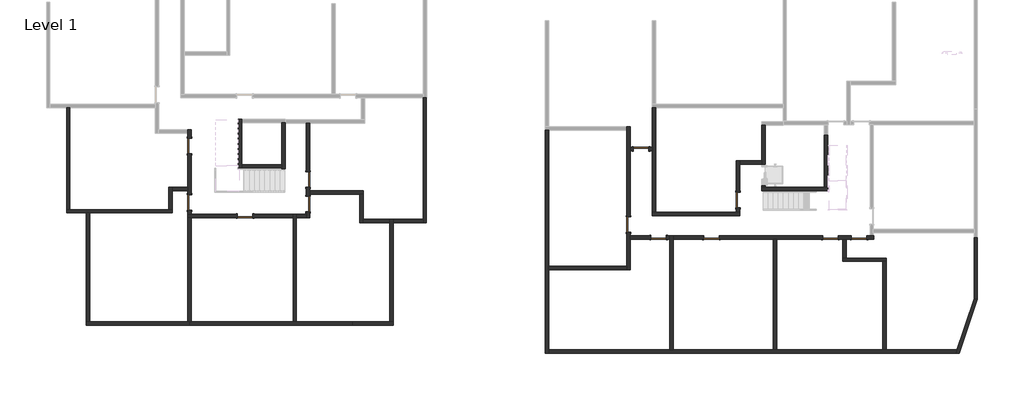
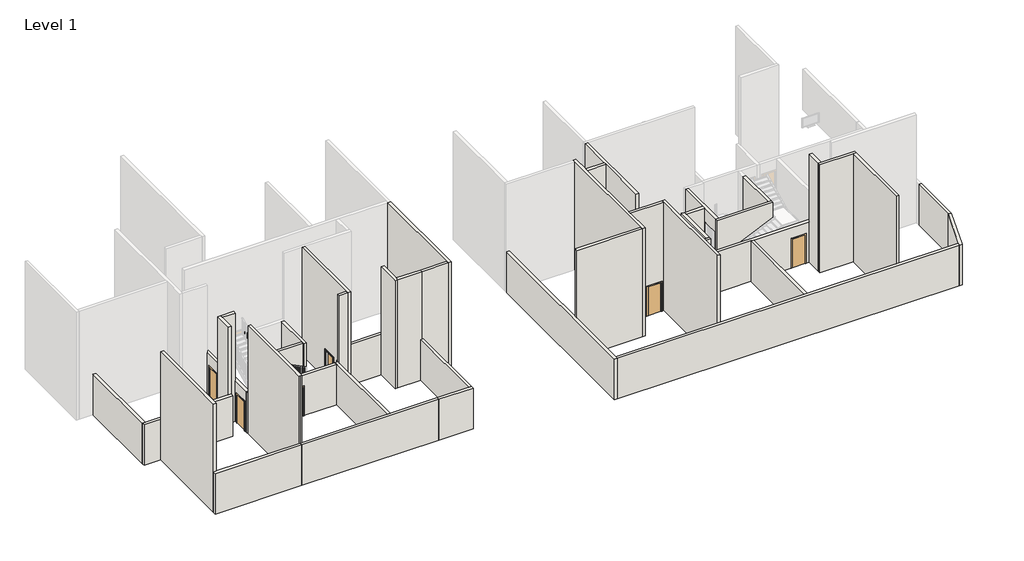
# One storey, part 1 of 3: 44 walls, 12 doors.
"""IFC4 building model written with IfcOpenShell, lengths in millimetres."""

import ifcopenshell
import ifcopenshell.guid

model = None  # the IFC model being written
_history = None  # IfcOwnerHistory: only IFC2X3 demands one
_inside = {}  # id of a spatial element -> (the spatial element, [elements in it])
_under = {}  # id of a project, library or spatial element -> (it, [spatial elements below it])
_declared = {}  # id of a project -> (the project, [libraries it declares])
_typed = {}  # id of a type object -> (the type object, [elements of that type])
_made_of = {}  # id of a material, layer set ... -> (it, [elements and type objects made of it])


def new_model(schema):
    """Start an empty IFC model of exactly this schema.

    Asked for "IFC4X3", IfcOpenShell would pick the latest addendum, in which some entities
    have other attributes; the version numbers below select the first issue.
    IFC2X3 requires an IfcOwnerHistory on every rooted entity: one is made here for all.
    """
    global model, _history
    if schema == "IFC4X3":
        model = ifcopenshell.file(schema_version=(4, 3, 0, 0))
    else:
        model = ifcopenshell.file(schema=schema)
    _inside.clear()
    _under.clear()
    _declared.clear()
    _typed.clear()
    _made_of.clear()
    _history = None
    if model.schema == "IFC2X3":
        org = make("IfcOrganization", Name="unknown")
        user = make(
            "IfcPersonAndOrganization",
            ThePerson=make("IfcPerson", FamilyName="unknown"),
            TheOrganization=org,
        )
        app = make(
            "IfcApplication",
            ApplicationDeveloper=org,
            Version="unknown",
            ApplicationFullName="unknown",
            ApplicationIdentifier="unknown",
        )
        _history = make(
            "IfcOwnerHistory",
            OwningUser=user,
            OwningApplication=app,
            ChangeAction="ADDED",
            CreationDate=0,
        )
    return model


def make(cls, **values):
    """One entity of the class cls with the attributes given. An attribute that is None is left unset."""
    return model.create_entity(
        cls, **{name: value for name, value in values.items() if value is not None}
    )


def rooted(cls, **values):
    """An entity with a GlobalId (a new one), such as an element, a storey or a relation."""
    return make(cls, GlobalId=ifcopenshell.guid.new(), OwnerHistory=_history, **values)


def si_unit(unit_type, name, prefix=None):
    """IfcSIUnit, for example si_unit("LENGTHUNIT", "METRE", prefix="MILLI")."""
    return make("IfcSIUnit", UnitType=unit_type, Prefix=prefix, Name=name)


def assignment(units):
    """IfcUnitAssignment: the units of a project."""
    return None if units is None else make("IfcUnitAssignment", Units=units)


def point(xyz):
    """IfcCartesianPoint."""
    return None if xyz is None else make("IfcCartesianPoint", Coordinates=xyz)


def direction(xyz):
    """IfcDirection."""
    return None if xyz is None else make("IfcDirection", DirectionRatios=xyz)


def frame(location, z_axis=None, x_axis=None):
    """IfcAxis2Placement3D, a coordinate frame: its origin and axes. An axis left out is left unset."""
    return make(
        "IfcAxis2Placement3D",
        Location=point(location),
        Axis=direction(z_axis),
        RefDirection=direction(x_axis),
    )


def origin():
    """The frame at (0, 0, 0) with its axes left unset."""
    return frame((0.0, 0.0, 0.0))


def origin_with_axes():
    """The frame at (0, 0, 0) with the z axis (0, 0, 1) and the x axis (1, 0, 0) written out."""
    return frame((0.0, 0.0, 0.0), z_axis=(0.0, 0.0, 1.0), x_axis=(1.0, 0.0, 0.0))


def place(relative_to, where):
    """IfcLocalPlacement: puts the frame where relative to a parent placement (None: the world)."""
    return make(
        "IfcLocalPlacement", PlacementRelTo=relative_to, RelativePlacement=where
    )


def context(
    kind, dimensions, precision=None, world=None, true_north=None, identifier=None
):
    """IfcGeometricRepresentationContext, for example the 3D "Model" context."""
    return make(
        "IfcGeometricRepresentationContext",
        ContextIdentifier=identifier,
        ContextType=kind,
        CoordinateSpaceDimension=dimensions,
        Precision=precision,
        WorldCoordinateSystem=world,
        TrueNorth=true_north,
    )


def project(units=None, contexts=None):
    """IfcProject with its units and contexts."""
    return rooted(
        "IfcProject",
        Name="project",
        RepresentationContexts=contexts,
        UnitsInContext=assignment(units),
    )


def spatial(cls, under=None, at=None, **own):
    """A site, building, storey or space (cls), placed at a placement, below another one or the project."""
    s = rooted(cls, ObjectPlacement=at, **own)
    if under is not None:
        _under.setdefault(under.id(), (under, []))[1].append(s)
    return s


def polyline(points):
    """IfcPolyline through the points."""
    return make("IfcPolyline", Points=[point(p) for p in points])


def outline(outer, holes=None, kind="AREA"):
    """IfcArbitraryClosedProfileDef: a profile drawn as a closed curve; with holes, ...WithVoids."""
    if holes is None:
        return make("IfcArbitraryClosedProfileDef", ProfileType=kind, OuterCurve=outer)
    return make(
        "IfcArbitraryProfileDefWithVoids",
        ProfileType=kind,
        OuterCurve=outer,
        InnerCurves=holes,
    )


def extrude(swept, where, along, depth):
    """IfcExtrudedAreaSolid: the profile swept, set in the frame where, extruded along a direction by depth."""
    return make(
        "IfcExtrudedAreaSolid",
        SweptArea=swept,
        Position=where,
        ExtrudedDirection=direction(along),
        Depth=depth,
    )


def faces_of(points, faces, orient=None, outer=None):
    """IfcFace entities. A face is a list of loops; a loop is a list of indices into points, from 0.

    orient and outer hold one flag for each loop. By default every Orientation is true, the
    first loop of a face is its IfcFaceOuterBound and the others are IfcFaceBound.
    """
    made = []
    for i, loops in enumerate(faces):
        bounds = []
        for j, loop in enumerate(loops):
            is_outer = j == 0 if outer is None else outer[i][j]
            bounds.append(
                make(
                    "IfcFaceOuterBound" if is_outer else "IfcFaceBound",
                    Bound=make("IfcPolyLoop", Polygon=[points[k] for k in loop]),
                    Orientation=True if orient is None else orient[i][j],
                )
            )
        made.append(make("IfcFace", Bounds=bounds))
    return made


def faceted_brep(points, faces, orient=None, outer=None, voids=None):
    """IfcFacetedBrep: a solid bounded by flat faces; with voids (closed shells), ...WithVoids."""
    shared = [point(p) for p in points]
    hull = make("IfcClosedShell", CfsFaces=faces_of(shared, faces, orient, outer))
    if voids is None:
        return make("IfcFacetedBrep", Outer=hull)
    return make(
        "IfcFacetedBrepWithVoids",
        Outer=hull,
        Voids=[
            make(cls, CfsFaces=faces_of(shared, fs, o, b)) for cls, fs, o, b in voids
        ],
    )


def shape(context_of_items, identifier, shape_type, items):
    """IfcShapeRepresentation: the items that make up one representation, for example the "Body"."""
    return make(
        "IfcShapeRepresentation",
        ContextOfItems=context_of_items,
        RepresentationIdentifier=identifier,
        RepresentationType=shape_type,
        Items=items,
    )


def source(mapping_origin, context_of_items, identifier, shape_type, items):
    """IfcRepresentationMap: a shape defined once, which mapped items show again and again."""
    return make(
        "IfcRepresentationMap",
        MappingOrigin=mapping_origin,
        MappedRepresentation=shape(context_of_items, identifier, shape_type, items),
    )


def transform(
    local_origin,
    x_axis=None,
    y_axis=None,
    z_axis=None,
    scale=None,
    scale2=None,
    scale3=None,
    uniform=True,
):
    """IfcCartesianTransformationOperator3D, or its non-uniform kind. x_axis, y_axis, z_axis: its Axis1, 2, 3."""
    if uniform:
        return make(
            "IfcCartesianTransformationOperator3D",
            Axis1=direction(x_axis),
            Axis2=direction(y_axis),
            LocalOrigin=point(local_origin),
            Scale=scale,
            Axis3=direction(z_axis),
        )
    return make(
        "IfcCartesianTransformationOperator3DnonUniform",
        Axis1=direction(x_axis),
        Axis2=direction(y_axis),
        LocalOrigin=point(local_origin),
        Scale=scale,
        Axis3=direction(z_axis),
        Scale2=scale2,
        Scale3=scale3,
    )


def mapped(mapping_source, mapping_target):
    """IfcMappedItem: shows the shape of a source again, moved by a transform."""
    return make(
        "IfcMappedItem", MappingSource=mapping_source, MappingTarget=mapping_target
    )


def made_of(thing, what):
    """Note that an element or type object is made of a material, layer set ...; save() writes the relation."""
    if what is not None:
        _made_of.setdefault(what.id(), (what, []))[1].append(thing)
    return thing


def element(
    cls,
    number,
    at=None,
    inside=None,
    cuts=None,
    type_object=None,
    material=None,
    context=None,
    identifier="Body",
    shape_type=None,
    held_by="IfcProductDefinitionShape",
    body=None,
    shapes=None,
    **own,
):
    """One element of the class cls, such as IfcWall. Its Tag is "e" and its number.

    at: its placement. inside: the storey or other place that contains it. cuts: it is an
    opening in that element (IfcRelVoidsElement). A single representation is given by context,
    identifier, shape_type and body (its items); several are given by shapes. held_by: the class
    of the entity that holds the representations. save() writes the other relations.
    """
    e = rooted(cls, Tag="e%d" % number, ObjectPlacement=at, **own)
    if body is not None:
        shapes = [shape(context, identifier, shape_type, body)]
    if shapes is not None:
        e.Representation = make(held_by, Representations=shapes)
    if inside is not None:
        _inside.setdefault(inside.id(), (inside, []))[1].append(e)
    if cuts is not None:
        rooted(
            "IfcRelVoidsElement", RelatingBuildingElement=cuts, RelatedOpeningElement=e
        )
    if type_object is not None:
        _typed.setdefault(type_object.id(), (type_object, []))[1].append(e)
    return made_of(e, material)


def aggregate(whole, parts):
    """IfcRelAggregates: a whole, such as a stair, and the parts it consists of."""
    return rooted("IfcRelAggregates", RelatingObject=whole, RelatedObjects=parts)


def save(model, path):
    """Write the relations noted so far, then the file.

    IfcRelAggregates (storeys below a building ...), IfcRelContainedInSpatialStructure (elements
    in a storey), IfcRelDefinesByType, IfcRelAssociatesMaterial and IfcRelDeclares: one each for
    every whole, place, type object, material and project.
    """
    for whole, parts in _under.values():
        aggregate(whole, parts)
    for where, things in _inside.values():
        rooted(
            "IfcRelContainedInSpatialStructure",
            RelatedElements=things,
            RelatingStructure=where,
        )
    for kind, things in _typed.values():
        rooted("IfcRelDefinesByType", RelatedObjects=things, RelatingType=kind)
    for what, things in _made_of.values():
        rooted("IfcRelAssociatesMaterial", RelatedObjects=things, RelatingMaterial=what)
    for by, libraries in _declared.values():
        rooted("IfcRelDeclares", RelatingContext=by, RelatedDefinitions=libraries)
    model.write(path)


def m_single_flush_0915_x_2134mm_727434cd(model_context):
    return source(origin(), model_context, "Body", "SweptSolid", [
        extrude(outline(polyline([(2210.0, -533.5), (0.0, -533.5), (0.0, -457.5), (2134.0, -457.5), (2134.0, 457.5), (0.0, 457.5), (0.0, 533.5), (2210.0, 533.5), (2210.0, -533.5)])), frame((0.0, -125.0, 0.0), z_axis=(0.0, 1.0, 0.0), x_axis=(0.0, 0.0, 1.0)), (0.0, 0.0, 1.0), 25.0),
        extrude(outline(polyline([(2210.0, 533.5), (2210.0, -533.5), (0.0, -533.5), (0.0, -457.5), (2134.0, -457.5), (2134.0, 457.5), (0.0, 457.5), (0.0, 533.5), (2210.0, 533.5)])), frame((0.0, 100.0, 0.0), z_axis=(0.0, 1.0, 0.0), x_axis=(0.0, 0.0, 1.0)), (0.0, 0.0, 1.0), 25.0),
        extrude(outline(polyline([(457.5, -49.0), (457.5, -100.0), (-457.5, -100.0), (-457.5, -49.0), (457.5, -49.0)])), origin_with_axes(), (0.0, 0.0, 1.0), 2134.0),
    ])


def m_single_flush_0915_x_2134mm_6a9e8738(model_context):
    return source(origin(), model_context, "Body", "SweptSolid", [
        extrude(outline(polyline([(2210.0, -533.5), (0.0, -533.5), (0.0, -457.5), (2134.0, -457.5), (2134.0, 457.5), (0.0, 457.5), (0.0, 533.5), (2210.0, 533.5), (2210.0, -533.5)])), frame((0.0, 100.0, 0.0), z_axis=(0.0, 1.0, 0.0), x_axis=(0.0, 0.0, 1.0)), (0.0, 0.0, 1.0), 25.0),
        extrude(outline(polyline([(2210.0, 533.5), (2210.0, -533.5), (0.0, -533.5), (0.0, -457.5), (2134.0, -457.5), (2134.0, 457.5), (0.0, 457.5), (0.0, 533.5), (2210.0, 533.5)])), frame((0.0, -125.0, 0.0), z_axis=(0.0, 1.0, 0.0), x_axis=(0.0, 0.0, 1.0)), (0.0, 0.0, 1.0), 25.0),
        extrude(outline(polyline([(457.5, 49.0), (-457.5, 49.0), (-457.5, 100.0), (457.5, 100.0), (457.5, 49.0)])), origin_with_axes(), (0.0, 0.0, 1.0), 2134.0),
    ])


model = new_model("IFC4")

# Units and contexts
model_context = context("Model", 3, world=origin())
ifc_project = project(units=[si_unit("LENGTHUNIT", "METRE", prefix="MILLI")], contexts=[model_context])

# Site, building, storey
site = spatial("IfcSite", under=ifc_project)
building = spatial("IfcBuilding", under=site)
storey = spatial("IfcBuildingStorey", under=building, Name="Level 1", Elevation=0.0)

# Doors
placement = place(None, origin())
m_single_flush_0915_x_2134mm_shape = m_single_flush_0915_x_2134mm_727434cd(model_context)
element("IfcDoor", 1, ObjectType="M_Single-Flush : 0915 x 2134mm", at=placement, inside=storey, context=model_context, shape_type="MappedRepresentation", body=[
    mapped(m_single_flush_0915_x_2134mm_shape, transform((16170.6041014, -4023.024372, 0.0), x_axis=(0.0, -1.0, 0.0), y_axis=(1.0, 0.0, 0.0), z_axis=(0.0, 0.0, 1.0))),
])
element("IfcDoor", 2, ObjectType="M_Single-Flush : 0915 x 2134mm", at=placement, inside=storey, context=model_context, shape_type="MappedRepresentation", body=[
    mapped(m_single_flush_0915_x_2134mm_shape, transform((-9130.3629108, -4269.650264, 0.0), x_axis=(0.0, 1.0, 0.0), y_axis=(-1.0, 0.0, 0.0), z_axis=(0.0, 0.0, 1.0))),
])
element("IfcDoor", 3, ObjectType="M_Single-Flush : 0915 x 2134mm", at=placement, inside=storey, context=model_context, shape_type="MappedRepresentation", body=[
    mapped(m_single_flush_0915_x_2134mm_shape, transform((9728.8612349, -5479.1907835, 0.0), x_axis=(0.0, -1.0, 0.0), y_axis=(1.0, 0.0, 0.0), z_axis=(0.0, 0.0, 1.0))),
])
element("IfcDoor", 4, ObjectType="M_Single-Flush : 0915 x 2134mm", at=placement, inside=storey, context=model_context, shape_type="MappedRepresentation", body=[
    mapped(m_single_flush_0915_x_2134mm_shape, transform((21611.3612349, -6240.0098119, 0.0), x_axis=(1.0, 0.0, 0.0), y_axis=(0.0, 1.0, 0.0), z_axis=(0.0, 0.0, 1.0))),
])
element("IfcDoor", 5, ObjectType="M_Single-Flush : 0915 x 2134mm", at=placement, inside=storey, context=model_context, shape_type="MappedRepresentation", body=[
    mapped(m_single_flush_0915_x_2134mm_shape, transform((11502.336337, -6236.6907835, 0.0), x_axis=(1.0, 0.0, 0.0), y_axis=(0.0, 1.0, 0.0), z_axis=(0.0, 0.0, 1.0))),
])
m_single_flush_0915_x_2134mm_2_shape = m_single_flush_0915_x_2134mm_6a9e8738(model_context)
element("IfcDoor", 6, ObjectType="M_Single-Flush : 0915 x 2134mm", at=placement, inside=storey, context=model_context, shape_type="MappedRepresentation", body=[
    mapped(m_single_flush_0915_x_2134mm_2_shape, transform((14602.336337, -6240.0098119, 0.0), x_axis=(-1.0, 0.0, 0.0), y_axis=(0.0, -1.0, 0.0), z_axis=(0.0, 0.0, 1.0))),
])
element("IfcDoor", 7, ObjectType="M_Single-Flush : 0915 x 2134mm", at=placement, inside=storey, context=model_context, shape_type="MappedRepresentation", body=[
    mapped(m_single_flush_0915_x_2134mm_2_shape, transform((23308.8612349, -6240.0098119, 0.0), x_axis=(-1.0, 0.0, 0.0), y_axis=(0.0, -1.0, 0.0), z_axis=(0.0, 0.0, 1.0))),
])
element("IfcDoor", 8, ObjectType="M_Single-Flush : 0915 x 2134mm", at=placement, inside=storey, context=model_context, shape_type="MappedRepresentation", body=[
    mapped(m_single_flush_0915_x_2134mm_2_shape, transform((-12832.3304233, -4959.1627129, 0.0), x_axis=(-1.0, 0.0, 0.0), y_axis=(0.0, -1.0, 0.0), z_axis=(0.0, 0.0, 1.0))),
])
element("IfcDoor", 9, ObjectType="M_Single-Flush : 0915 x 2134mm", at=placement, inside=storey, context=model_context, shape_type="MappedRepresentation", body=[
    mapped(m_single_flush_0915_x_2134mm_2_shape, transform((-16113.9741722, -844.6599715, 0.0), x_axis=(0.0, 1.0, 0.0), y_axis=(-1.0, 0.0, 0.0), z_axis=(0.0, 0.0, 1.0))),
])
element("IfcDoor", 10, ObjectType="M_Single-Flush : 0915 x 2134mm", at=placement, inside=storey, context=model_context, shape_type="MappedRepresentation", body=[
    mapped(m_single_flush_0915_x_2134mm_2_shape, transform((-16113.9741722, -4173.1613422, 0.0), x_axis=(0.0, 1.0, 0.0), y_axis=(-1.0, 0.0, 0.0), z_axis=(0.0, 0.0, 1.0))),
])
element("IfcDoor", 11, ObjectType="M_Single-Flush : 0915 x 2134mm", at=placement, inside=storey, context=model_context, shape_type="MappedRepresentation", body=[
    mapped(m_single_flush_0915_x_2134mm_2_shape, transform((-9130.3629108, -2822.6378151, 0.0), x_axis=(0.0, -1.0, 0.0), y_axis=(1.0, 0.0, 0.0), z_axis=(0.0, 0.0, 1.0))),
])
element("IfcDoor", 12, ObjectType="M_Single-Flush : 0915 x 2134mm", at=placement, inside=storey, context=model_context, shape_type="MappedRepresentation", body=[
    mapped(m_single_flush_0915_x_2134mm_2_shape, transform((10478.8612349, -1020.524372, 0.0), x_axis=(1.0, 0.0, 0.0), y_axis=(0.0, 1.0, 0.0), z_axis=(0.0, 0.0, 1.0))),
])

# Walls
element("IfcWall", 13, ObjectType="Generic - 200mm", at=placement, inside=storey, context=model_context, shape_type="Brep", body=[
    faceted_brep([(30069.3799498, -6240.0098119, 0.0), (30069.3799498, -9831.8731192, 0.0), (30069.3799498, -9831.8731192, 3000.0), (30069.3799498, -6240.0098119, 3000.0), (30269.3799498, -6240.0098119, 0.0), (30269.3799498, -6240.0098119, 3000.0), (30269.3799498, -9864.7113693, 3000.0), (30269.3799498, -9864.7113693, 0.0), (30268.8612349, -6240.0098119, 0.0), (30268.8612349, -6240.0098119, 3000.0)], [[[0, 1, 2, 3]], [[4, 5, 6, 7]], [[1, 0, 8, 4, 7]], [[3, 2, 6, 5, 9]], [[0, 3, 9, 5, 4, 8]], [[2, 1, 7, 6]]]),
])
element("IfcWall", 14, ObjectType="Generic - 200mm", at=placement, inside=storey, context=model_context, shape_type="Brep", body=[
    faceted_brep([(21449.836337, -3276.2808257, 0.0), (21249.836337, -3276.2808257, 0.0), (17770.6041014, -3276.2808257, 0.0), (17570.6041014, -3276.2808257, 0.0), (17570.6041014, -3276.2808257, 3000.0), (17770.6041014, -3276.2808257, 3000.0), (21249.836337, -3276.2808257, 3000.0), (21449.836337, -3276.2808257, 3000.0), (21449.836337, -3476.2808257, 0.0), (21449.836337, -3476.2808257, 3000.0), (17570.6041014, -3476.2808257, 3000.0), (17570.6041014, -3476.2808257, 0.0)], [[[0, 1, 2, 3, 4, 5, 6, 7]], [[8, 9, 10, 11]], [[3, 2, 1, 0, 8, 11]], [[7, 6, 5, 4, 10, 9]], [[0, 7, 9, 8]], [[4, 3, 11, 10]]]),
])
element("IfcWall", 15, ObjectType="Generic - 200mm", at=placement, inside=storey, context=model_context, shape_type="SweptSolid", body=[
    extrude(outline(polyline([(18459.836337, -6340.0098119), (18459.836337, -12836.6907835), (18259.836337, -12836.6907835), (18259.836337, -6340.0098119), (18459.836337, -6340.0098119)])), origin_with_axes(), (0.0, 0.0, 1.0), 3000.0),
])
element("IfcWall", 16, ObjectType="Generic - 200mm", at=placement, inside=storey, context=model_context, shape_type="Brep", body=[
    faceted_brep([(29055.3124022, -12836.6907835, 0.0), (24888.8612349, -12836.6907835, 0.0), (24688.8612349, -12836.6907835, 0.0), (18459.836337, -12836.6907835, 0.0), (18259.836337, -12836.6907835, 0.0), (12359.836337, -12836.6907835, 0.0), (12159.836337, -12836.6907835, 0.0), (5043.716007, -12836.6907835, 0.0), (5043.716007, -12836.6907835, 3000.0), (18259.836337, -12836.6907835, 3000.0), (18459.836337, -12836.6907835, 3000.0), (29055.3124022, -12836.6907835, 3000.0), (28987.8162902, -13036.6907835, 0.0), (28987.8162902, -13036.6907835, 3000.0), (5043.716007, -13036.6907835, 3000.0), (5043.716007, -13036.6907835, 0.0)], [[[0, 1, 2, 3, 4, 5, 6, 7, 8, 9, 10, 11]], [[12, 13, 14, 15]], [[7, 6, 5, 4, 3, 2, 1, 0, 12, 15]], [[11, 10, 9, 8, 14, 13]], [[0, 11, 13, 12]], [[8, 7, 15, 14]]]),
])
element("IfcWall", 17, ObjectType="Generic - 200mm", at=placement, inside=storey, context=model_context, shape_type="Brep", body=[
    faceted_brep([(30069.3799498, -9831.8731192, 0.0), (29055.3124022, -12836.6907835, 0.0), (28987.8162902, -13036.6907835, 0.0), (28987.8162902, -13036.6907835, 3000.0), (29055.3124022, -12836.6907835, 3000.0), (30069.3799498, -9831.8731192, 3000.0), (30269.3799498, -9864.7113693, 0.0), (30269.3799498, -9864.7113693, 3000.0), (29198.8985612, -13036.6907835, 3000.0), (29198.8985612, -13036.6907835, 0.0)], [[[0, 1, 2, 3, 4, 5]], [[6, 7, 8, 9]], [[2, 1, 0, 6, 9]], [[5, 4, 3, 8, 7]], [[0, 5, 7, 6]], [[3, 2, 9, 8]]]),
])
element("IfcWall", 18, ObjectType="Generic - 200mm", at=placement, inside=storey, context=model_context, shape_type="Brep", body=[
    faceted_brep([(22851.3612349, -6140.0098119, 0.0), (22068.8612349, -6140.0098119, 0.0), (22068.8612349, -6140.0098119, 2134.0), (21153.8612349, -6140.0098119, 2134.0), (21153.8612349, -6140.0098119, 0.0), (15059.836337, -6140.0098119, 0.0), (15059.836337, -6140.0098119, 2134.0), (14144.836337, -6140.0098119, 2134.0), (14144.836337, -6140.0098119, 0.0), (12359.836337, -6140.0098119, 0.0), (12359.836337, -6140.0098119, 3000.0), (23948.8612349, -6140.0098119, 3000.0), (24148.8612349, -6140.0098119, 3000.0), (24163.3998354, -6140.0098119, 3000.0), (24163.3998354, -6140.0098119, 0.0), (24148.8612349, -6140.0098119, 0.0), (23948.8612349, -6140.0098119, 0.0), (23766.3612349, -6140.0098119, 0.0), (23766.3612349, -6140.0098119, 2134.0), (22851.3612349, -6140.0098119, 2134.0), (22068.8612349, -6340.0098119, 2134.0), (22068.8612349, -6340.0098119, 0.0), (22348.8612349, -6340.0098119, 0.0), (22548.8612349, -6340.0098119, 0.0), (22851.3612349, -6340.0098119, 0.0), (22851.3612349, -6340.0098119, 2134.0), (23766.3612349, -6340.0098119, 2134.0), (23766.3612349, -6340.0098119, 0.0), (24163.3998354, -6340.0098119, 0.0), (24163.3998354, -6340.0098119, 3000.0), (18459.836337, -6340.0098119, 3000.0), (18259.836337, -6340.0098119, 3000.0), (12359.836337, -6340.0098119, 3000.0), (12359.836337, -6340.0098119, 0.0), (14144.836337, -6340.0098119, 0.0), (14144.836337, -6340.0098119, 2134.0), (15059.836337, -6340.0098119, 2134.0), (15059.836337, -6340.0098119, 0.0), (18259.836337, -6340.0098119, 0.0), (18459.836337, -6340.0098119, 0.0), (21153.8612349, -6340.0098119, 0.0), (21153.8612349, -6340.0098119, 2134.0)], [[[0, 1, 2, 3, 4, 5, 6, 7, 8, 9, 10, 11, 12, 13, 14, 15, 16, 17, 18, 19]], [[20, 21, 22, 23, 24, 25, 26, 27, 28, 29, 30, 31, 32, 33, 34, 35, 36, 37, 38, 39, 40, 41]], [[33, 9, 8, 34]], [[17, 16, 15, 14, 28, 27]], [[40, 39, 38, 37, 5, 4]], [[24, 23, 22, 21, 1, 0]], [[13, 12, 11, 10, 32, 31, 30, 29]], [[14, 13, 29, 28]], [[7, 35, 34, 8]], [[36, 6, 5, 37]], [[6, 36, 35, 7]], [[25, 24, 0, 19]], [[26, 25, 19, 18]], [[27, 26, 18, 17]], [[10, 9, 33, 32]], [[2, 1, 21, 20]], [[3, 2, 20, 41]], [[4, 3, 41, 40]]]),
])
element("IfcWall", 19, ObjectType="Generic - 200mm", at=placement, inside=storey, context=model_context, shape_type="Brep", body=[
    faceted_brep([(4843.716007, 79.9901881, 0.0), (4843.716007, -13036.6907835, 0.0), (4843.716007, -13036.6907835, 3000.0), (4843.716007, 79.9901881, 3000.0), (5043.716007, 79.9901881, 0.0), (5043.716007, 79.9901881, 3000.0), (5043.716007, -12836.6907835, 3000.0), (5043.716007, -13036.6907835, 3000.0), (5043.716007, -13036.6907835, 0.0), (5043.716007, -12836.6907835, 0.0), (5043.716007, -8120.0098119, 0.0), (5043.716007, -7920.0098119, 0.0)], [[[0, 1, 2, 3]], [[4, 5, 6, 7, 8, 9, 10, 11]], [[1, 0, 4, 11, 10, 9, 8]], [[3, 2, 7, 6, 5]], [[2, 1, 8, 7]], [[0, 3, 5, 4]]]),
])
element("IfcWall", 20, ObjectType="Generic - 200mm", at=placement, inside=storey, context=model_context, shape_type="SweptSolid", body=[
    extrude(outline(polyline([(21249.836337, -3276.2808257), (21249.836337, -200.524372), (21449.836337, -200.524372), (21449.836337, -3276.2808257), (21249.836337, -3276.2808257)])), origin_with_axes(), (0.0, 0.0, 1.0), 3000.0),
])
element("IfcWall", 21, ObjectType="Generic - 200mm", at=placement, inside=storey, context=model_context, shape_type="Brep", body=[
    faceted_brep([(17570.6041014, -3276.2808257, 3000.0), (17570.6041014, -1920.524372, 3000.0), (17570.6041014, -1720.524372, 3000.0), (17570.6041014, 379.475628, 3000.0), (17570.6041014, 379.475628, 0.0), (17570.6041014, -1720.524372, 0.0), (17570.6041014, -1920.524372, 0.0), (17570.6041014, -1926.2808257, 0.0), (17570.6041014, -1926.2808257, 2000.0), (17570.6041014, -3181.2876228, 2000.0), (17570.6041014, -3181.2876228, 0.0), (17570.6041014, -3276.2808257, 0.0), (17770.6041014, 379.475628, 3000.0), (17770.6041014, -3276.2808257, 3000.0), (17770.6041014, -3276.2808257, 0.0), (17770.6041014, -3181.2876228, 0.0), (17770.6041014, -3181.2876228, 2000.0), (17770.6041014, -1926.2808257, 2000.0), (17770.6041014, -1926.2808257, 0.0), (17770.6041014, 379.475628, 0.0)], [[[0, 1, 2, 3, 4, 5, 6, 7, 8, 9, 10, 11]], [[12, 13, 14, 15, 16, 17, 18, 19]], [[14, 11, 10, 15]], [[4, 19, 18, 7, 6, 5]], [[3, 2, 1, 0, 13, 12]], [[0, 11, 14, 13]], [[9, 16, 15, 10]], [[17, 8, 7, 18]], [[8, 17, 16, 9]], [[4, 3, 12, 19]]]),
])
element("IfcWall", 22, ObjectType="Generic - 200mm", at=placement, inside=storey, context=model_context, shape_type="Brep", body=[
    faceted_brep([(11128.8612349, -4940.0098119, 0.0), (16270.6041014, -4940.0098119, 0.0), (16270.6041014, -4940.0098119, 3000.0), (11128.8612349, -4940.0098119, 3000.0), (11128.8612349, -4740.0098119, 0.0), (11128.8612349, -4740.0098119, 3000.0), (16070.6041014, -4740.0098119, 3000.0), (16270.6041014, -4740.0098119, 3000.0), (16270.6041014, -4740.0098119, 0.0), (16070.6041014, -4740.0098119, 0.0), (11328.8612349, -4740.0098119, 0.0)], [[[0, 1, 2, 3]], [[4, 5, 6, 7, 8, 9, 10]], [[1, 0, 4, 10, 9, 8]], [[3, 2, 7, 6, 5]], [[2, 1, 8, 7]], [[0, 3, 5, 4]]]),
])
element("IfcWall", 23, ObjectType="Generic - 200mm", at=placement, inside=storey, context=model_context, shape_type="Brep", body=[
    faceted_brep([(16270.6041014, -1720.524372, 3000.0), (16270.6041014, -1920.524372, 3000.0), (16270.6041014, -4740.0098119, 3000.0), (16270.6041014, -4740.0098119, 0.0), (16270.6041014, -4480.524372, 0.0), (16270.6041014, -4480.524372, 2134.0), (16270.6041014, -3565.524372, 2134.0), (16270.6041014, -3565.524372, 0.0), (16270.6041014, -1920.524372, 0.0), (16270.6041014, -1720.524372, 0.0), (16070.6041014, -4740.0098119, 3000.0), (16070.6041014, -1720.524372, 3000.0), (16070.6041014, -1720.524372, 0.0), (16070.6041014, -3565.524372, 0.0), (16070.6041014, -3565.524372, 2134.0), (16070.6041014, -4480.524372, 2134.0), (16070.6041014, -4480.524372, 0.0), (16070.6041014, -4740.0098119, 0.0)], [[[0, 1, 2, 3, 4, 5, 6, 7, 8, 9]], [[10, 11, 12, 13, 14, 15, 16, 17]], [[3, 17, 16, 4]], [[12, 9, 8, 7, 13]], [[2, 1, 0, 11, 10]], [[3, 2, 10, 17]], [[0, 9, 12, 11]], [[15, 5, 4, 16]], [[6, 14, 13, 7]], [[14, 6, 5, 15]]]),
])
element("IfcWall", 24, ObjectType="Generic - 200mm", at=placement, inside=storey, context=model_context, shape_type="SweptSolid", body=[
    extrude(outline(polyline([(17570.6041014, -1920.524372), (16270.6041014, -1920.524372), (16270.6041014, -1720.524372), (17570.6041014, -1720.524372), (17570.6041014, -1920.524372)])), origin_with_axes(), (0.0, 0.0, 1.0), 3000.0),
])
element("IfcWall", 25, ObjectType="Generic - 200mm", at=placement, inside=storey, context=model_context, shape_type="Brep", body=[
    faceted_brep([(22348.8612349, -7641.2808257, 0.0), (24688.8612349, -7641.2808257, 0.0), (24888.8612349, -7641.2808257, 0.0), (24888.8612349, -7641.2808257, 8000.0), (24688.8612349, -7641.2808257, 8000.0), (22348.8612349, -7641.2808257, 8000.0), (22348.8612349, -7441.2808257, 0.0), (22348.8612349, -7441.2808257, 8000.0), (22548.8612349, -7441.2808257, 8000.0), (24888.8612349, -7441.2808257, 8000.0), (24888.8612349, -7441.2808257, 0.0), (22548.8612349, -7441.2808257, 0.0)], [[[0, 1, 2, 3, 4, 5]], [[6, 7, 8, 9, 10, 11]], [[2, 1, 0, 6, 11, 10]], [[5, 4, 3, 9, 8, 7]], [[3, 2, 10, 9]], [[0, 5, 7, 6]]]),
])
element("IfcWall", 26, ObjectType="Generic - 200mm", at=placement, inside=storey, context=model_context, shape_type="SweptSolid", body=[
    extrude(outline(polyline([(24688.8612349, -12836.6907835), (24688.8612349, -7641.2808257), (24888.8612349, -7641.2808257), (24888.8612349, -12836.6907835), (24688.8612349, -12836.6907835)])), origin_with_axes(), (0.0, 0.0, 1.0), 8000.0),
])
element("IfcWall", 27, ObjectType="Generic - 200mm", at=placement, inside=storey, context=model_context, shape_type="SweptSolid", body=[
    extrude(outline(polyline([(22548.8612349, -6340.0098119), (22548.8612349, -7441.2808257), (22348.8612349, -7441.2808257), (22348.8612349, -6340.0098119), (22548.8612349, -6340.0098119)])), origin_with_axes(), (0.0, 0.0, 1.0), 8000.0),
])
element("IfcWall", 28, ObjectType="Generic - 200mm", at=placement, inside=storey, context=model_context, shape_type="Brep", body=[
    faceted_brep([(9628.8612349, -5936.6907835, 2134.0), (9628.8612349, -5936.6907835, 0.0), (9628.8612349, -7920.0098119, 0.0), (9628.8612349, -8120.0098119, 0.0), (9628.8612349, -8120.0098119, 8000.0), (9628.8612349, -7920.0098119, 8000.0), (9628.8612349, 79.9901881, 8000.0), (9628.8612349, 279.9901881, 8000.0), (9628.8612349, 279.9901881, 0.0), (9628.8612349, 79.9901881, 0.0), (9628.8612349, -5021.6907835, 0.0), (9628.8612349, -5021.6907835, 2134.0), (9828.8612349, -8120.0098119, 0.0), (9828.8612349, -6336.6907835, 0.0), (9828.8612349, -6136.6907835, 0.0), (9828.8612349, -5936.6907835, 0.0), (9828.8612349, -5936.6907835, 2134.0), (9828.8612349, -5021.6907835, 2134.0), (9828.8612349, -5021.6907835, 0.0), (9828.8612349, -1120.524372, 0.0), (9828.8612349, -920.524372, 0.0), (9828.8612349, 279.9901881, 0.0), (9828.8612349, 279.9901881, 8000.0), (9828.8612349, -920.524372, 8000.0), (9828.8612349, -1120.524372, 8000.0), (9828.8612349, -6136.6907835, 8000.0), (9828.8612349, -6336.6907835, 8000.0), (9828.8612349, -8120.0098119, 8000.0)], [[[0, 1, 2, 3, 4, 5, 6, 7, 8, 9, 10, 11]], [[12, 13, 14, 15, 16, 17, 18, 19, 20, 21, 22, 23, 24, 25, 26, 27]], [[10, 9, 8, 21, 20, 19, 18]], [[3, 2, 1, 15, 14, 13, 12]], [[7, 6, 5, 4, 27, 26, 25, 24, 23, 22]], [[8, 7, 22, 21]], [[4, 3, 12, 27]], [[16, 15, 1, 0]], [[17, 16, 0, 11]], [[18, 17, 11, 10]]]),
])
element("IfcWall", 29, ObjectType="Generic - 200mm", at=placement, inside=storey, context=model_context, shape_type="SweptSolid", body=[
    extrude(outline(polyline([(5043.716007, -7920.0098119), (9628.8612349, -7920.0098119), (9628.8612349, -8120.0098119), (5043.716007, -8120.0098119), (5043.716007, -7920.0098119)])), origin_with_axes(), (0.0, 0.0, 1.0), 8000.0),
])
element("IfcWall", 30, ObjectType="Generic - 200mm", at=placement, inside=storey, context=model_context, shape_type="Brep", body=[
    faceted_brep([(-4309.8304233, -5158.643998, 0.0), (-4309.8304233, -5358.643998, 0.0), (-4309.8304233, -11188.643998, 0.0), (-4309.8304233, -11188.643998, 3000.0), (-4309.8304233, -5358.643998, 3000.0), (-4309.8304233, -5158.643998, 3000.0), (-4109.8304233, -5158.643998, 0.0), (-4109.8304233, -5158.643998, 3000.0), (-4109.8304233, -5358.643998, 3000.0), (-4109.8304233, -11188.643998, 3000.0), (-4109.8304233, -11188.643998, 0.0), (-4109.8304233, -5358.643998, 0.0), (-4209.8304233, -5158.643998, 3000.0)], [[[0, 1, 2, 3, 4, 5]], [[6, 7, 8, 9, 10, 11]], [[2, 1, 0, 6, 11, 10]], [[5, 4, 3, 9, 8, 7, 12]], [[3, 2, 10, 9]], [[0, 5, 12, 7, 6]]]),
])
element("IfcWall", 31, ObjectType="Generic - 200mm", at=placement, inside=storey, context=model_context, shape_type="Brep", body=[
    faceted_brep([(-4109.8304233, -11188.643998, 0.0), (-4309.8304233, -11188.643998, 0.0), (-6530.3449834, -11188.643998, 0.0), (-6530.3449834, -11188.643998, 3000.0), (-4309.8304233, -11188.643998, 3000.0), (-4109.8304233, -11188.643998, 3000.0), (-4109.8304233, -11388.643998, 0.0), (-4109.8304233, -11388.643998, 3000.0), (-6530.3449834, -11388.643998, 3000.0), (-6530.3449834, -11388.643998, 0.0), (-6530.3449834, -11189.1627129, 0.0), (-6530.3449834, -11189.1627129, 3000.0)], [[[0, 1, 2, 3, 4, 5]], [[6, 7, 8, 9]], [[2, 1, 0, 6, 9, 10]], [[3, 2, 10, 9, 8, 11]], [[5, 4, 3, 11, 8, 7]], [[0, 5, 7, 6]]]),
])
element("IfcWall", 32, ObjectType="Generic - 200mm", at=placement, inside=storey, context=model_context, shape_type="Brep", body=[
    faceted_brep([(-6530.3449834, -11189.1627129, 0.0), (-9814.8304233, -11189.1627129, 0.0), (-10014.8304233, -11189.1627129, 0.0), (-16014.8304233, -11189.1627129, 0.0), (-16114.8304233, -11189.1627129, 0.0), (-16114.8304233, -11189.1627129, 3000.0), (-10014.8304233, -11189.1627129, 3000.0), (-9814.8304233, -11189.1627129, 3000.0), (-6530.3449834, -11189.1627129, 3000.0), (-6530.3449834, -11389.1627129, 0.0), (-6530.3449834, -11389.1627129, 3000.0), (-16114.8304233, -11389.1627129, 3000.0), (-16114.8304233, -11389.1627129, 0.0), (-6530.3449834, -11388.643998, 0.0), (-16114.8304233, -11189.6814279, 0.0), (-16114.8304233, -11189.6814279, 3000.0), (-6530.3449834, -11388.643998, 3000.0)], [[[0, 1, 2, 3, 4, 5, 6, 7, 8]], [[9, 10, 11, 12]], [[4, 3, 2, 1, 0, 13, 9, 12, 14]], [[5, 4, 14, 12, 11, 15]], [[8, 7, 6, 5, 15, 11, 10, 16]], [[0, 8, 16, 10, 9, 13]]]),
])
element("IfcWall", 33, ObjectType="Generic - 200mm", at=placement, inside=storey, context=model_context, shape_type="Brep", body=[
    faceted_brep([(-16114.8304233, -11189.6814279, 0.0), (-16214.8304233, -11189.6814279, 0.0), (-21985.6447259, -11189.6814279, 0.0), (-22185.6447259, -11189.6814279, 0.0), (-22185.6447259, -11189.6814279, 3000.0), (-16114.8304233, -11189.6814279, 3000.0), (-16114.8304233, -11389.6814279, 0.0), (-16114.8304233, -11389.6814279, 3000.0), (-22185.6447259, -11389.6814279, 3000.0), (-22185.6447259, -11389.6814279, 0.0), (-16114.8304233, -11389.1627129, 0.0), (-16114.8304233, -11389.1627129, 3000.0)], [[[0, 1, 2, 3, 4, 5]], [[6, 7, 8, 9]], [[3, 2, 1, 0, 10, 6, 9]], [[5, 4, 8, 7, 11]], [[0, 5, 11, 7, 6, 10]], [[4, 3, 9, 8]]]),
])
element("IfcWall", 34, ObjectType="Generic - 200mm", at=placement, inside=storey, context=model_context, shape_type="Brep", body=[
    faceted_brep([(-13026.101437, -2140.1378151, 0.0), (-13026.101437, -1940.1378151, 0.0), (-13026.101437, 520.8372871, 0.0), (-13026.101437, 720.8372871, 0.0), (-13026.101437, 720.8372871, 3000.0), (-13026.101437, 520.8372871, 3000.0), (-13026.101437, -1940.1378151, 3000.0), (-13026.101437, -2140.1378151, 3000.0), (-13226.101437, -2140.1378151, 0.0), (-13226.101437, -2140.1378151, 3000.0), (-13226.101437, 720.8372871, 3000.0), (-13226.101437, 720.8372871, 0.0)], [[[0, 1, 2, 3, 4, 5, 6, 7]], [[8, 9, 10, 11]], [[3, 2, 1, 0, 8, 11]], [[7, 6, 5, 4, 10, 9]], [[0, 7, 9, 8]], [[4, 3, 11, 10]]]),
])
element("IfcWall", 35, ObjectType="Generic - 200mm", at=placement, inside=storey, context=model_context, shape_type="Brep", body=[
    faceted_brep([(-23346.5113948, -4787.1599715, 0.0), (-22185.6447259, -4787.1599715, 0.0), (-21985.6447259, -4787.1599715, 0.0), (-17123.9741722, -4787.1599715, 0.0), (-17123.9741722, -4787.1599715, 3000.0), (-23346.5113948, -4787.1599715, 3000.0), (-23346.5113948, -4587.1599715, 0.0), (-23346.5113948, -4587.1599715, 3000.0), (-23146.5113948, -4587.1599715, 3000.0), (-17123.9741722, -4587.1599715, 3000.0), (-17123.9741722, -4587.1599715, 0.0), (-17323.9741722, -4587.1599715, 0.0), (-23146.5113948, -4587.1599715, 0.0)], [[[0, 1, 2, 3, 4, 5]], [[6, 7, 8, 9, 10, 11, 12]], [[3, 2, 1, 0, 6, 12, 11, 10]], [[4, 3, 10, 9]], [[5, 4, 9, 8, 7]], [[0, 5, 7, 6]]]),
])
element("IfcWall", 36, ObjectType="Generic - 200mm", at=placement, inside=storey, context=model_context, shape_type="SweptSolid", body=[
    extrude(outline(polyline([(-23146.5113948, 1412.8400285), (-23146.5113948, -4587.1599715), (-23346.5113948, -4587.1599715), (-23346.5113948, 1412.8400285), (-23146.5113948, 1412.8400285)])), origin_with_axes(), (0.0, 0.0, 1.0), 3000.0),
])
element("IfcWall", 37, ObjectType="Generic - 200mm", at=placement, inside=storey, context=model_context, shape_type="Brep", body=[
    faceted_brep([(-16013.9741722, -3715.6613422, 2134.0), (-16013.9741722, -3715.6613422, 0.0), (-16013.9741722, -1302.1599715, 0.0), (-16013.9741722, -1302.1599715, 2134.0), (-16013.9741722, -387.1599715, 2134.0), (-16013.9741722, -387.1599715, 0.0), (-16013.9741722, 112.8400285, 0.0), (-16013.9741722, 112.8400285, 3000.0), (-16013.9741722, -4859.1627129, 3000.0), (-16013.9741722, -4859.1627129, 0.0), (-16013.9741722, -4630.6613422, 0.0), (-16013.9741722, -4630.6613422, 2134.0), (-16213.9741722, -1302.1599715, 0.0), (-16213.9741722, -3287.1599715, 0.0), (-16213.9741722, -3487.1599715, 0.0), (-16213.9741722, -3715.6613422, 0.0), (-16213.9741722, -3715.6613422, 2134.0), (-16213.9741722, -4630.6613422, 2134.0), (-16213.9741722, -4630.6613422, 0.0), (-16213.9741722, -4859.1627129, 0.0), (-16213.9741722, -4859.1627129, 3000.0), (-16213.9741722, 112.8400285, 3000.0), (-16213.9741722, 112.8400285, 0.0), (-16213.9741722, -87.1599715, 0.0), (-16213.9741722, -387.1599715, 0.0), (-16213.9741722, -387.1599715, 2134.0), (-16213.9741722, -1302.1599715, 2134.0)], [[[0, 1, 2, 3, 4, 5, 6, 7, 8, 9, 10, 11]], [[12, 13, 14, 15, 16, 17, 18, 19, 20, 21, 22, 23, 24, 25, 26]], [[6, 5, 24, 23, 22]], [[10, 9, 19, 18]], [[2, 1, 15, 14, 13, 12]], [[8, 7, 21, 20]], [[7, 6, 22, 21]], [[9, 8, 20, 19]], [[25, 24, 5, 4]], [[26, 25, 4, 3]], [[12, 26, 3, 2]], [[16, 15, 1, 0]], [[17, 16, 0, 11]], [[18, 17, 11, 10]]]),
])
element("IfcWall", 38, ObjectType="Generic - 200mm", at=placement, inside=storey, context=model_context, shape_type="Brep", body=[
    faceted_brep([(-10014.8304233, -5059.1627129, 3000.0), (-16213.9741722, -5059.1627129, 3000.0), (-16213.9741722, -5059.1627129, 0.0), (-16014.8304233, -5059.1627129, 0.0), (-13289.8304233, -5059.1627129, 0.0), (-13289.8304233, -5059.1627129, 2134.0), (-12374.8304233, -5059.1627129, 2134.0), (-12374.8304233, -5059.1627129, 0.0), (-10014.8304233, -5059.1627129, 0.0), (-16213.9741722, -4859.1627129, 3000.0), (-16013.9741722, -4859.1627129, 3000.0), (-10014.8304233, -4859.1627129, 3000.0), (-10014.8304233, -4859.1627129, 0.0), (-12374.8304233, -4859.1627129, 0.0), (-12374.8304233, -4859.1627129, 2134.0), (-13289.8304233, -4859.1627129, 2134.0), (-13289.8304233, -4859.1627129, 0.0), (-16013.9741722, -4859.1627129, 0.0), (-16213.9741722, -4859.1627129, 0.0)], [[[0, 1, 2, 3, 4, 5, 6, 7, 8]], [[9, 10, 11, 12, 13, 14, 15, 16, 17, 18]], [[12, 8, 7, 13]], [[2, 18, 17, 16, 4, 3]], [[1, 0, 11, 10, 9]], [[0, 8, 12, 11]], [[15, 5, 4, 16]], [[6, 14, 13, 7]], [[14, 6, 5, 15]], [[2, 1, 9, 18]]]),
])
element("IfcWall", 39, ObjectType="Generic - 200mm", at=placement, inside=storey, context=model_context, shape_type="SweptSolid", body=[
    extrude(outline(polyline([(-13026.101437, -1940.1378151), (-10669.8304233, -1940.1378151), (-10669.8304233, -2140.1378151), (-13026.101437, -2140.1378151), (-13026.101437, -1940.1378151)])), origin_with_axes(), (0.0, 0.0, 1.0), 3000.0),
])
element("IfcWall", 40, ObjectType="Generic - 200mm", at=placement, inside=storey, context=model_context, shape_type="Brep", body=[
    faceted_brep([(-9030.3629108, -3680.1378151, 0.0), (-6095.3449834, -3680.1378151, 0.0), (-5895.3449834, -3680.1378151, 0.0), (-5895.3449834, -3680.1378151, 3000.0), (-9030.3629108, -3680.1378151, 3000.0), (-9030.3629108, -3480.1378151, 0.0), (-9030.3629108, -3480.1378151, 3000.0), (-5895.3449834, -3480.1378151, 3000.0), (-5895.3449834, -3480.1378151, 0.0)], [[[0, 1, 2, 3, 4]], [[5, 6, 7, 8]], [[2, 1, 0, 5, 8]], [[4, 3, 7, 6]], [[3, 2, 8, 7]], [[0, 4, 6, 5]]]),
])
element("IfcWall", 41, ObjectType="Generic - 200mm", at=placement, inside=storey, context=model_context, shape_type="Brep", body=[
    faceted_brep([(-10014.8304233, -4859.1627129, 0.0), (-10014.8304233, -5059.1627129, 0.0), (-10014.8304233, -11189.1627129, 0.0), (-10014.8304233, -11189.1627129, 3000.0), (-10014.8304233, -5059.1627129, 3000.0), (-10014.8304233, -4859.1627129, 3000.0), (-9814.8304233, -4859.1627129, 0.0), (-9814.8304233, -4859.1627129, 3000.0), (-9814.8304233, -11189.1627129, 3000.0), (-9814.8304233, -11189.1627129, 0.0), (-9814.8304233, -5059.1627129, 0.0)], [[[0, 1, 2, 3, 4, 5]], [[6, 7, 8, 9, 10]], [[2, 1, 0, 6, 10, 9]], [[5, 4, 3, 8, 7]], [[3, 2, 9, 8]], [[0, 5, 7, 6]]]),
])
element("IfcWall", 42, ObjectType="Generic - 200mm", at=placement, inside=storey, context=model_context, shape_type="Brep", body=[
    faceted_brep([(-10469.8304233, -2179.1627129, 0.0), (-10469.8304233, 500.8372871, 0.0), (-10469.8304233, 520.8372871, 0.0), (-10469.8304233, 520.8372871, 3000.0), (-10469.8304233, -2179.1627129, 3000.0), (-10669.8304233, -2179.1627129, 0.0), (-10669.8304233, -2179.1627129, 3000.0), (-10669.8304233, -2140.1378151, 3000.0), (-10669.8304233, -1940.1378151, 3000.0), (-10669.8304233, 520.8372871, 3000.0), (-10669.8304233, 520.8372871, 0.0), (-10669.8304233, -1940.1378151, 0.0), (-10669.8304233, -2140.1378151, 0.0)], [[[0, 1, 2, 3, 4]], [[5, 6, 7, 8, 9, 10, 11, 12]], [[2, 1, 0, 5, 12, 11, 10]], [[4, 3, 9, 8, 7, 6]], [[0, 4, 6, 5]], [[3, 2, 10, 9]]]),
])
element("IfcWall", 43, ObjectType="Generic - 200mm", at=placement, inside=storey, context=model_context, shape_type="Brep", body=[
    faceted_brep([(-6095.3449834, -3680.1378151, 0.0), (-6095.3449834, -5358.643998, 0.0), (-6095.3449834, -5358.643998, 8000.0), (-6095.3449834, -3680.1378151, 8000.0), (-5895.3449834, -3680.1378151, 0.0), (-5895.3449834, -3680.1378151, 3000.0), (-5895.3449834, -3680.1378151, 8000.0), (-5895.3449834, -5158.643998, 8000.0), (-5895.3449834, -5358.643998, 8000.0), (-5895.3449834, -5358.643998, 0.0), (-5895.3449834, -5158.643998, 0.0)], [[[0, 1, 2, 3]], [[4, 5, 6, 7, 8, 9, 10]], [[1, 0, 4, 10, 9]], [[3, 2, 8, 7, 6]], [[2, 1, 9, 8]], [[0, 3, 6, 5, 4]]]),
])
element("IfcWall", 44, ObjectType="Generic - 200mm", at=placement, inside=storey, context=model_context, shape_type="SweptSolid", body=[
    extrude(outline(polyline([(0.0, -5895.3449834), (0.0, -4309.8304233), (3000.0, -4309.8304233), (3000.0, -4209.8304233), (8000.0, -4209.8304233), (8000.0, -5895.3449834), (0.0, -5895.3449834)])), frame((0.0, -5358.643998, 0.0), z_axis=(0.0, 1.0, 0.0), x_axis=(0.0, 0.0, 1.0)), (0.0, 0.0, 1.0), 200.0),
])
element("IfcWall", 45, ObjectType="Generic - 200mm", at=placement, inside=storey, context=model_context, shape_type="Brep", body=[
    faceted_brep([(12159.836337, -6136.6907835, 0.0), (12159.836337, -6336.6907835, 0.0), (12159.836337, -12836.6907835, 0.0), (12159.836337, -12836.6907835, 8000.0), (12159.836337, -6336.6907835, 8000.0), (12159.836337, -6136.6907835, 8000.0), (12359.836337, -6136.6907835, 0.0), (12359.836337, -6136.6907835, 8000.0), (12359.836337, -12836.6907835, 8000.0), (12359.836337, -12836.6907835, 0.0), (12359.836337, -6340.0098119, 0.0), (12359.836337, -6140.0098119, 0.0)], [[[0, 1, 2, 3, 4, 5]], [[6, 7, 8, 9, 10, 11]], [[2, 1, 0, 6, 11, 10, 9]], [[5, 4, 3, 8, 7]], [[3, 2, 9, 8]], [[0, 5, 7, 6]]]),
])
element("IfcWall", 46, ObjectType="Generic - 200mm", at=placement, inside=storey, context=model_context, shape_type="SweptSolid", body=[
    extrude(outline(polyline([(2134.0, 11959.836337), (0.0, 11959.836337), (0.0, 12159.836337), (8000.0, 12159.836337), (8000.0, 9828.8612349), (0.0, 9828.8612349), (0.0, 11044.836337), (2134.0, 11044.836337), (2134.0, 11959.836337)])), frame((0.0, -6336.6907835, 0.0), z_axis=(0.0, 1.0, 0.0), x_axis=(0.0, 0.0, 1.0)), (0.0, 0.0, 1.0), 200.0),
])
element("IfcWall", 47, ObjectType="Generic - 200mm", at=placement, inside=storey, context=model_context, shape_type="SweptSolid", body=[
    extrude(outline(polyline([(0.0, -4109.8304233), (0.0, -2360.3449834), (8000.0, -2360.3449834), (8000.0, -4209.8304233), (3000.0, -4209.8304233), (3000.0, -4109.8304233), (0.0, -4109.8304233)])), frame((0.0, -5358.643998, 0.0), z_axis=(0.0, 1.0, 0.0), x_axis=(0.0, 0.0, 1.0)), (0.0, 0.0, 1.0), 200.0),
])
element("IfcWall", 48, ObjectType="Generic - 200mm", at=placement, inside=storey, context=model_context, shape_type="Brep", body=[
    faceted_brep([(-16214.8304233, -5059.1627129, 0.0), (-16214.8304233, -11189.6814279, 0.0), (-16214.8304233, -11189.6814279, 8000.0), (-16214.8304233, -5059.1627129, 8000.0), (-16014.8304233, -5059.1627129, 0.0), (-16014.8304233, -5059.1627129, 8000.0), (-16014.8304233, -11189.1627129, 8000.0), (-16014.8304233, -11189.1627129, 0.0), (-16213.9741722, -5059.1627129, 0.0), (-16114.8304233, -11189.1627129, 0.0), (-16114.8304233, -11189.6814279, 0.0), (-16114.8304233, -11189.6814279, 8000.0), (-16114.8304233, -11189.1627129, 8000.0), (-16114.8304233, -11189.6814279, 3000.0), (-16114.8304233, -11189.1627129, 3000.0)], [[[0, 1, 2, 3]], [[4, 5, 6, 7]], [[1, 0, 8, 4, 7, 9, 10]], [[3, 2, 11, 12, 6, 5]], [[2, 1, 10, 13, 11]], [[10, 9, 14, 12, 11, 13]], [[9, 7, 6, 12, 14]], [[0, 3, 5, 4, 8]]]),
])
element("IfcWall", 49, ObjectType="Generic - 200mm", at=placement, inside=storey, context=model_context, shape_type="Brep", body=[
    faceted_brep([(-21985.6447259, -11189.6814279, 0.0), (-21985.6447259, -4787.1599715, 0.0), (-21985.6447259, -4787.1599715, 8000.0), (-21985.6447259, -11189.6814279, 8000.0), (-22185.6447259, -11189.6814279, 0.0), (-22185.6447259, -11189.6814279, 3000.0), (-22185.6447259, -11189.6814279, 8000.0), (-22185.6447259, -4787.1599715, 8000.0), (-22185.6447259, -4787.1599715, 0.0)], [[[0, 1, 2, 3]], [[4, 5, 6, 7, 8]], [[1, 0, 4, 8]], [[3, 2, 7, 6]], [[2, 1, 8, 7]], [[0, 3, 6, 5, 4]]]),
])
element("IfcWall", 50, ObjectType="Generic - 200mm", at=placement, inside=storey, context=model_context, shape_type="Brep", body=[
    faceted_brep([(-2360.3449834, 2000.8372871, 0.0), (-2360.3449834, -5158.643998, 0.0), (-2360.3449834, -5358.643998, 0.0), (-2360.3449834, -5358.643998, 8000.0), (-2360.3449834, -5158.643998, 8000.0), (-2360.3449834, 2000.8372871, 8000.0), (-2160.3449834, 2000.8372871, 0.0), (-2160.3449834, 2000.8372871, 8000.0), (-2160.3449834, -5358.643998, 8000.0), (-2160.3449834, -5358.643998, 0.0), (-2350.3449834, 2000.8372871, 0.0), (-2350.3449834, 2000.8372871, 8000.0)], [[[0, 1, 2, 3, 4, 5]], [[6, 7, 8, 9]], [[2, 1, 0, 10, 6, 9]], [[5, 4, 3, 8, 7, 11]], [[3, 2, 9, 8]], [[0, 5, 11, 7, 6, 10]]]),
])
element("IfcWall", 51, ObjectType="Generic - 200mm", at=placement, inside=storey, context=model_context, shape_type="Brep", body=[
    faceted_brep([(-9230.3629108, -3280.1378151, 2134.0), (-9230.3629108, -3280.1378151, 0.0), (-9230.3629108, -3812.150264, 0.0), (-9230.3629108, -3812.150264, 2134.0), (-9230.3629108, -4727.150264, 2134.0), (-9230.3629108, -4727.150264, 0.0), (-9230.3629108, -4859.1627129, 0.0), (-9230.3629108, -5059.1627129, 0.0), (-9230.3629108, -5059.1627129, 8000.0), (-9230.3629108, -4859.1627129, 8000.0), (-9230.3629108, 500.8372871, 8000.0), (-9230.3629108, 500.8372871, 0.0), (-9230.3629108, -2365.1378151, 0.0), (-9230.3629108, -2365.1378151, 2134.0), (-9030.3629108, -3812.150264, 0.0), (-9030.3629108, -3680.1378151, 0.0), (-9030.3629108, -3480.1378151, 0.0), (-9030.3629108, -3280.1378151, 0.0), (-9030.3629108, -3280.1378151, 2134.0), (-9030.3629108, -2365.1378151, 2134.0), (-9030.3629108, -2365.1378151, 0.0), (-9030.3629108, 500.8372871, 0.0), (-9030.3629108, 500.8372871, 8000.0), (-9030.3629108, -5059.1627129, 8000.0), (-9030.3629108, -5059.1627129, 0.0), (-9030.3629108, -4727.150264, 0.0), (-9030.3629108, -4727.150264, 2134.0), (-9030.3629108, -3812.150264, 2134.0)], [[[0, 1, 2, 3, 4, 5, 6, 7, 8, 9, 10, 11, 12, 13]], [[14, 15, 16, 17, 18, 19, 20, 21, 22, 23, 24, 25, 26, 27]], [[25, 24, 7, 6, 5]], [[12, 11, 21, 20]], [[2, 1, 17, 16, 15, 14]], [[10, 9, 8, 23, 22]], [[11, 10, 22, 21]], [[8, 7, 24, 23]], [[3, 2, 14, 27]], [[4, 3, 27, 26]], [[5, 4, 26, 25]], [[18, 17, 1, 0]], [[19, 18, 0, 13]], [[20, 19, 13, 12]]]),
])
element("IfcWall", 52, ObjectType="Generic - 200mm", at=placement, inside=storey, context=model_context, shape_type="Brep", body=[
    faceted_brep([(-9814.8304233, -5059.1627129, 0.0), (-9230.3629108, -5059.1627129, 0.0), (-9230.3629108, -5059.1627129, 8000.0), (-9814.8304233, -5059.1627129, 8000.0), (-9814.8304233, -4859.1627129, 0.0), (-9814.8304233, -4859.1627129, 3000.0), (-9814.8304233, -4859.1627129, 8000.0), (-9230.3629108, -4859.1627129, 8000.0), (-9230.3629108, -4859.1627129, 0.0)], [[[0, 1, 2, 3]], [[4, 5, 6, 7, 8]], [[1, 0, 4, 8]], [[3, 2, 7, 6]], [[0, 3, 6, 5, 4]], [[2, 1, 8, 7]]]),
])
element("IfcWall", 53, ObjectType="Generic - 200mm", at=placement, inside=storey, context=model_context, shape_type="Brep", body=[
    faceted_brep([(11328.8612349, -4740.0098119, 0.0), (11328.8612349, 1419.475628, 0.0), (11328.8612349, 1419.475628, 8000.0), (11328.8612349, -4740.0098119, 8000.0), (11128.8612349, -4740.0098119, 0.0), (11128.8612349, -4740.0098119, 3000.0), (11128.8612349, -4740.0098119, 8000.0), (11128.8612349, -1120.524372, 8000.0), (11128.8612349, -920.524372, 8000.0), (11128.8612349, 1419.475628, 8000.0), (11128.8612349, 1419.475628, 0.0), (11128.8612349, -920.524372, 0.0), (11128.8612349, -1120.524372, 0.0)], [[[0, 1, 2, 3]], [[4, 5, 6, 7, 8, 9, 10, 11, 12]], [[1, 0, 4, 12, 11, 10]], [[3, 2, 9, 8, 7, 6]], [[0, 3, 6, 5, 4]], [[2, 1, 10, 9]]]),
])
element("IfcWall", 54, ObjectType="Generic - 200mm", at=placement, inside=storey, context=model_context, shape_type="SweptSolid", body=[
    extrude(outline(polyline([(2134.0, 10936.3612349), (0.0, 10936.3612349), (0.0, 11128.8612349), (8000.0, 11128.8612349), (8000.0, 9828.8612349), (0.0, 9828.8612349), (0.0, 10021.3612349), (2134.0, 10021.3612349), (2134.0, 10936.3612349)])), frame((0.0, -1120.524372, 0.0), z_axis=(0.0, 1.0, 0.0), x_axis=(0.0, 0.0, 1.0)), (0.0, 0.0, 1.0), 200.0),
])
element("IfcWall", 55, ObjectType="Generic - 200mm", at=placement, inside=storey, context=model_context, shape_type="Brep", body=[
    faceted_brep([(-17123.9741722, -4587.1599715, 0.0), (-17123.9741722, -3487.1599715, 0.0), (-17123.9741722, -3287.1599715, 0.0), (-17123.9741722, -3287.1599715, 8000.0), (-17123.9741722, -3487.1599715, 8000.0), (-17123.9741722, -4587.1599715, 8000.0), (-17123.9741722, -4587.1599715, 3000.0), (-17323.9741722, -4587.1599715, 0.0), (-17323.9741722, -4587.1599715, 8000.0), (-17323.9741722, -3287.1599715, 8000.0), (-17323.9741722, -3287.1599715, 0.0)], [[[0, 1, 2, 3, 4, 5, 6]], [[7, 8, 9, 10]], [[2, 1, 0, 7, 10]], [[5, 4, 3, 9, 8]], [[0, 6, 5, 8, 7]], [[3, 2, 10, 9]]]),
])
element("IfcWall", 56, ObjectType="Generic - 200mm", at=placement, inside=storey, context=model_context, shape_type="SweptSolid", body=[
    extrude(outline(polyline([(-16213.9741722, -3487.1599715), (-17123.9741722, -3487.1599715), (-17123.9741722, -3287.1599715), (-16213.9741722, -3287.1599715), (-16213.9741722, -3487.1599715)])), origin_with_axes(), (0.0, 0.0, 1.0), 8000.0),
])

save(model, "model.ifc")

# Revit data of these elements
# Project information
#   Project Issue Date = "Issue Date"
#   Project Status = "Project Status"
#   Client Name = "Owner"
#   Project Address = "Enter address here"
#   Project Name = "Project Name"
#   Project Number = "0001"
# Type "M_Single-Flush : 0915 x 2134mm"
#   Type Mark = "20"
#   Construction Type Id = "MDOOR"
#   Analytic Construction = "Metal"
#   Thickness = 5.1 cm
#   Thermal Resistance (R) = 0.270117 (m²·K)/W
#   Heat Transfer Coefficient (U) = 3.7021 W/(m²·K)
#   Height = 213.4 cm
#   Trim Projection Ext = 2.5 cm
#   Trim Projection Int = 2.5 cm
#   Trim Width = 7.6 cm
#   Width = 91.5 cm
#   Define Thermal Properties by = 1
#   Define Thermal Properties by = 1
#   Door Material = Door - Panel
#   Frame Material = Door - Frame
#   Visual Light Transmittance = 0
#   Solar Heat Gain Coefficient = 0
#   Function = (empty or 0)
#   Wall Closure = (empty or 0)
# Type "Generic - 200mm"
#   Layers, outside or top first: 20 cm no material (function 1)
# Elements 1, 2, 3, 4, 5, 6, 7, 8, 9, 10, 11, 12 (IfcDoor, "M_Single-Flush : 0915 x 2134mm")
#   Phase Created = New Construction
#   Materials on its faces: "Door - Frame", "Door - Panel"
# Elements 13, 14, 15, 16, 17, 18, 19, 20, 21, 22, 23, 24, 30, 31, 32, 33, 34, 35, 36, 37, 38, 39, 40, 41, 42 (IfcWall, "Generic - 200mm")
#   Top Offset = 0 cm
#   Base Offset = 0 cm
#   wall height = 300 cm
#   Phase Created = New Construction
#   Base Constraint = Level 1
#   Top Constraint = Level 2
#   Materials on its faces: "Default Wall"
# Elements 25, 26, 27, 28, 29, 43, 44, 45, 46, 47, 48, 49, 50, 51, 52, 53, 54, 55, 56 (IfcWall, "Generic - 200mm")
#   Top Offset = 0 cm
#   Base Offset = 0 cm
#   Unconnected Height = 800 cm
#   wall height = 800 cm
#   Phase Created = New Construction
#   Base Constraint = Level 1
#   Materials on its faces: "Default Wall"
# Materials
#   "Door - Panel": class "Wood", colour RGB 210 159 95, transparency 0, Cost = 0
#   "Door - Frame": class "Miscellaneous", colour RGB 118 70 51, transparency 0, Cost = 0
#   "Default Wall": class "Miscellaneous", colour RGB 128 128 128, transparency 0, Cost = 0
# Room, not placed, phase "New Construction", upper offset 0 cm, lower offset 0 cm
#   Number = "11"
#   Name = "Room"
# Room, not placed, phase "New Construction", upper offset 0 cm, lower offset 0 cm
#   Number = "12"
#   Name = "Room"
# Room, not placed, phase "New Construction", upper offset 0 cm, lower offset 0 cm
#   Number = "13"
#   Name = "Room"
# Room, not placed, phase "New Construction", upper offset 0 cm, lower offset 0 cm
#   Number = "14"
#   Name = "Room"
# Room, not placed, phase "New Construction", upper offset 0 cm, lower offset 0 cm
#   Number = "15"
#   Name = "Room"
# Room, not placed, phase "New Construction", upper offset 0 cm, lower offset 0 cm
#   Number = "16"
#   Name = "Room"
# Room, not placed, phase "New Construction", upper offset 0 cm, lower offset 0 cm
#   Number = "30"
#   Name = "Room"
# Room, not placed, phase "New Construction", upper offset 0 cm, lower offset 0 cm
#   Number = "31"
#   Name = "Room"
# Area, not placed, upper offset 0 cm, lower offset 0 cm
#   Number = "4"
#   Name = "Dere Parsel Toplam Alan"
# Room, not placed, phase "New Construction", upper offset 0 cm, lower offset 0 cm
#   Number = "106"
#   Name = "Room"
# Room, not placed, phase "New Construction", upper offset 0 cm, lower offset 0 cm
#   Number = "107"
#   Name = "Room"
# Room, not placed, phase "New Construction", upper offset 0 cm, lower offset 0 cm
#   Number = "109"
#   Name = "Room"
# Room, not placed, phase "New Construction", upper offset 0 cm, lower offset 0 cm
#   Number = "110"
#   Name = "7"
# Room, not placed, phase "New Construction", upper offset 0 cm, lower offset 0 cm
#   Number = "111"
#   Name = "8"
# Room, not placed, phase "New Construction", upper offset 0 cm, lower offset 0 cm
#   Number = "112"
#   Name = "9"
# Room, not placed, phase "New Construction", upper offset 0 cm, lower offset 0 cm
#   Number = "113"
#   Name = "1"
# Room, not placed, phase "New Construction", upper offset 0 cm, lower offset 0 cm
#   Number = "114"
#   Name = "5"
# Room, not placed, phase "New Construction", upper offset 0 cm, lower offset 0 cm
#   Number = "115"
#   Name = "2"
# Room, not placed, phase "New Construction", upper offset 0 cm, lower offset 0 cm
#   Number = "116"
#   Name = "4"
# Room at (-16235.351, -8218.051) mm, phase "New Construction", upper level "Level 1", upper offset 243.84 cm, lower offset 0 cm
#   Number = "117"
#   Name = "3"
# Room, not placed, phase "New Construction", upper offset 0 cm, lower offset 0 cm
#   Number = "118"
#   Name = "6"
# Room, not placed, phase "New Construction", upper offset 0 cm, lower offset 0 cm
#   Number = "17"
#   Name = "Room"
# Room, not placed, phase "New Construction", upper offset 0 cm, lower offset 0 cm
#   Number = "119"
#   Name = "Room"
# Room, not placed, phase "New Construction", upper offset 0 cm, lower offset 0 cm
#   Number = "120"
#   Name = "Room"
# Room, not placed, phase "New Construction", upper offset 0 cm, lower offset 0 cm
#   Number = "77"
#   Name = "7"
# Room at (11394.672, -1537.737) mm, phase "New Construction", upper level "Level 1", upper offset 243.84 cm, lower offset 0 cm
#   Number = "78"
#   Name = "8"
# Room at (21715.408, 3344.32) mm, phase "New Construction", upper level "Level 1", upper offset 243.84 cm, lower offset 0 cm
#   Number = "79"
#   Name = "9"
# Room at (24094.982, 1386.264) mm, phase "New Construction", upper level "Level 1", upper offset 243.84 cm, lower offset 0 cm
#   Number = "80"
#   Name = "1"
# Room, not placed, phase "New Construction", upper offset 0 cm, lower offset 0 cm
#   Number = "81"
#   Name = "Room"
# Room, not placed, phase "New Construction", upper offset 0 cm, lower offset 0 cm
#   Number = "82"
#   Name = "Room"
